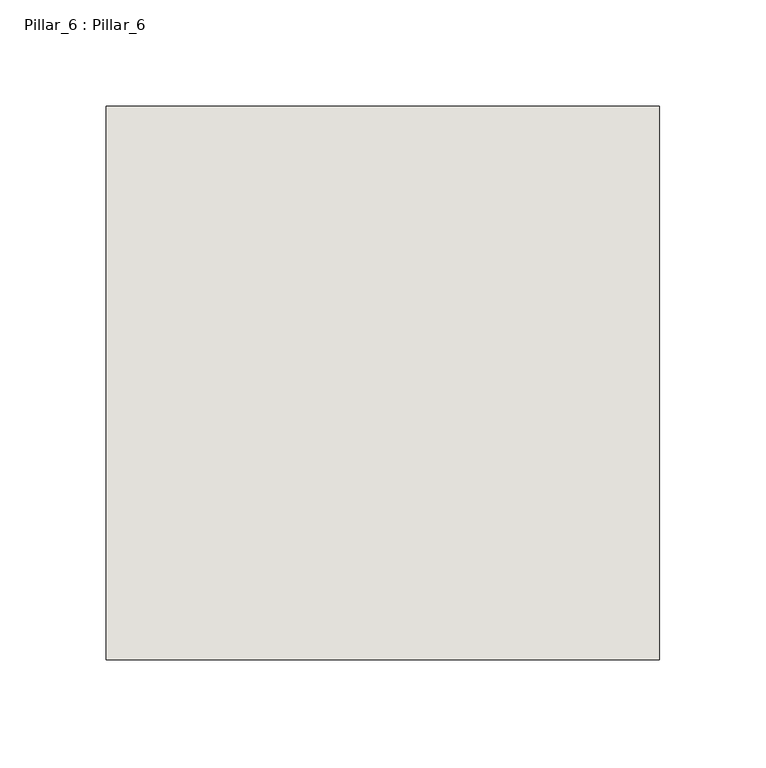
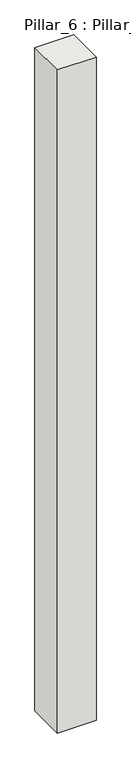
"""IFC4 building model written with IfcOpenShell, lengths in millimetres: wall geometry, Pillar_6 : Pillar_6."""

from ifc_helpers import new_model, si_unit, origin, origin_with_axes, place, context, project, spatial, polyline, outline, extrude, source, transform, mapped, element, save


def pillar_6_pillar_6_704e6477(model_context):
    return source(origin(), model_context, "Body", "SweptSolid", [
        extrude(outline(polyline([(2660.0, 16730.0), (2400.0, 16730.0), (2400.0, 16990.0), (2660.0, 16990.0), (2660.0, 16730.0)])), origin_with_axes(), (0.0, 0.0, 1.0), 4700.0),
    ])


if __name__ == "__main__":
    model = new_model("IFC4")
    model_context = context("Model", 3, world=origin())
    ifc_project = project(units=[si_unit("LENGTHUNIT", "METRE", prefix="MILLI")], contexts=[model_context])
    site = spatial("IfcSite", under=ifc_project)
    building = spatial("IfcBuilding", under=site)
    placement = place(None, origin())
    pillar_6_pillar_6_shape = pillar_6_pillar_6_704e6477(model_context)
    element("IfcWall", 1, ObjectType="Pillar_6 : Pillar_6", at=placement, inside=building, context=model_context, shape_type="MappedRepresentation", body=[
        mapped(pillar_6_pillar_6_shape, transform((0.0, 0.0, 0.0), x_axis=(1.0, 0.0, 0.0), y_axis=(0.0, 1.0, 0.0), z_axis=(0.0, 0.0, 1.0))),
    ])
    save(model, "model.ifc")

# Revit data of these elements
# Type "Pillar_6 : Pillar_6"
#   NameOverride = "Pillar_6"
# Element 1 (IfcWall, "Pillar_6 : Pillar_6")
#   Materials on its faces: "IfcSurfaceStyle #33"
# Materials
#   "IfcSurfaceStyle #33": class "Unassigned", colour RGB 214 214 214, transparency 0
